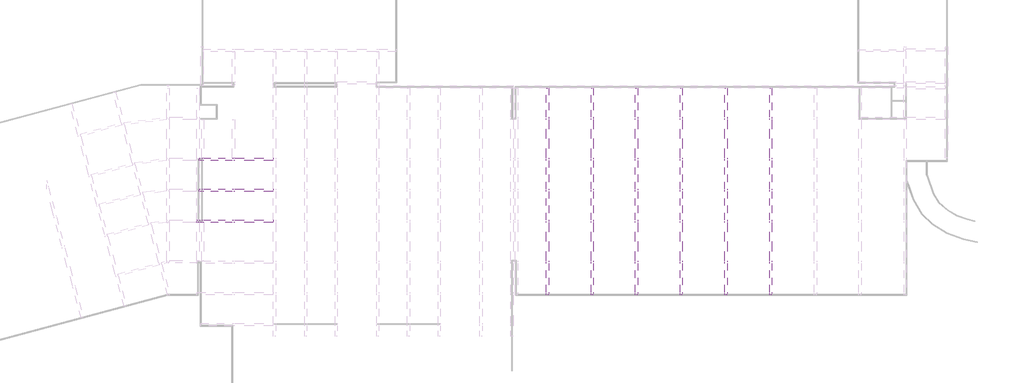
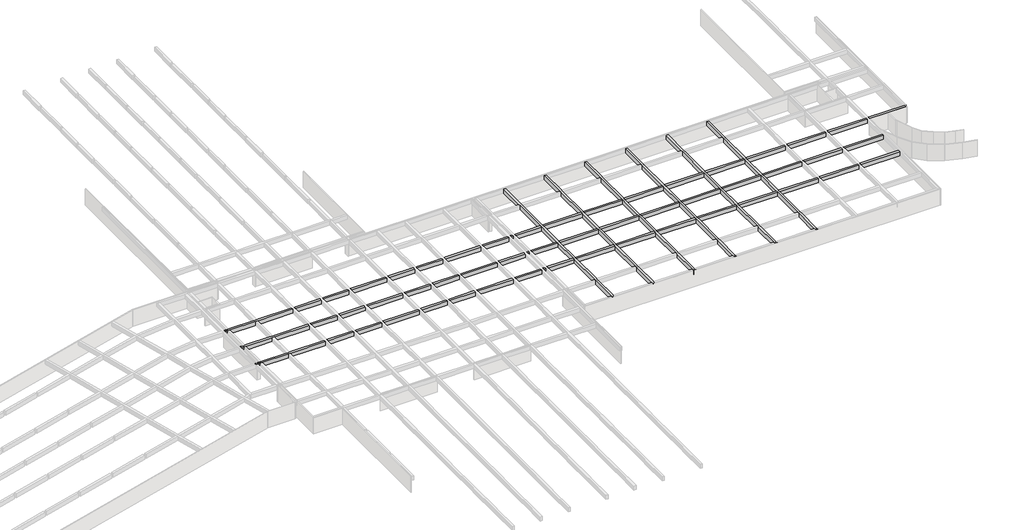
# One storey, part 9 of 14: 9 beams.
"""IFC4 building model written with IfcOpenShell, lengths in millimetres."""

from ifc_helpers import new_model, si_unit, origin, place, context, project, spatial, faceted_brep, element, save

model = new_model("IFC4")

# Units and contexts
model_context = context("Model", 3, world=origin())
ifc_project = project(units=[si_unit("LENGTHUNIT", "METRE", prefix="MILLI")], contexts=[model_context])

# Site, building, storey
site = spatial("IfcSite", under=ifc_project)
building = spatial("IfcBuilding", under=site)
storey = spatial("IfcBuildingStorey", under=building, Name="户型图", Elevation=0.0)

# Beams
placement = place(None, origin())
element("IfcBeam", 1, ObjectType="混凝土 - 矩形梁 : KL_beam", at=placement, inside=storey, context=model_context, shape_type="Brep", body=[
    faceted_brep([(73979.8514216, -218258.950757, 3300.0), (73579.8514216, -218258.950757, 3300.0), (73579.8514216, -218258.950757, 2500.0), (73979.8514216, -218258.950757, 2500.0), (73979.8514216, -218208.950757, 3300.0), (73979.8514216, -217808.950757, 3300.0), (73979.8514216, -212708.950757, 3300.0), (73979.8514216, -212308.950757, 3300.0), (73979.8514216, -205576.1028577, 3300.0), (73979.8514216, -205176.1028577, 3300.0), (73979.8514216, -200154.952508, 3300.0), (73979.8514216, -199754.952508, 3300.0), (73979.8514216, -194741.3993539, 3300.0), (73979.8514216, -194341.3993539, 3300.0), (73979.8514216, -187598.950757, 3300.0), (73979.8514216, -187198.950757, 3300.0), (73979.8514216, -182068.950757, 3300.0), (73579.8514216, -182068.950757, 3300.0), (73579.8514216, -187198.950757, 3300.0), (73579.8514216, -187598.950757, 3300.0), (73579.8514216, -194341.3993539, 3300.0), (73579.8514216, -194741.3993539, 3300.0), (73579.8514216, -199754.952508, 3300.0), (73579.8514216, -200154.952508, 3300.0), (73579.8514216, -205176.1028577, 3300.0), (73579.8514216, -205576.1028577, 3300.0), (73579.8514216, -212308.950757, 3300.0), (73579.8514216, -212708.950757, 3300.0), (73579.8514216, -217808.950757, 3300.0), (73579.8514216, -218208.950757, 3300.0), (73579.8514216, -182068.950757, 2500.0), (73579.8514216, -187198.950757, 2500.0), (73579.8514216, -187598.950757, 2500.0), (73579.8514216, -194341.3993539, 2500.0), (73579.8514216, -194741.3993539, 2500.0), (73579.8514216, -199754.952508, 2500.0), (73579.8514216, -200154.952508, 2500.0), (73579.8514216, -205176.1028577, 2500.0), (73579.8514216, -205576.1028577, 2500.0), (73579.8514216, -212308.950757, 2500.0), (73579.8514216, -212708.950757, 2500.0), (73579.8514216, -217808.950757, 2500.0), (73579.8514216, -218208.950757, 2500.0), (73979.8514216, -182068.950757, 2500.0), (73979.8514216, -187198.950757, 2500.0), (73979.8514216, -187598.950757, 2500.0), (73979.8514216, -194341.3993539, 2500.0), (73979.8514216, -194741.3993539, 2500.0), (73979.8514216, -199754.952508, 2500.0), (73979.8514216, -200154.952508, 2500.0), (73979.8514216, -205176.1028577, 2500.0), (73979.8514216, -205576.1028577, 2500.0), (73979.8514216, -212308.950757, 2500.0), (73979.8514216, -212708.950757, 2500.0), (73979.8514216, -217808.950757, 2500.0), (73979.8514216, -218208.950757, 2500.0)], [[[0, 1, 2, 3]], [[1, 0, 4, 5, 6, 7, 8, 9, 10, 11, 12, 13, 14, 15, 16, 17, 18, 19, 20, 21, 22, 23, 24, 25, 26, 27, 28, 29]], [[2, 1, 29, 28, 27, 26, 25, 24, 23, 22, 21, 20, 19, 18, 17, 30, 31, 32, 33, 34, 35, 36, 37, 38, 39, 40, 41, 42]], [[3, 2, 42, 41, 40, 39, 38, 37, 36, 35, 34, 33, 32, 31, 30, 43, 44, 45, 46, 47, 48, 49, 50, 51, 52, 53, 54, 55]], [[0, 3, 55, 54, 53, 52, 51, 50, 49, 48, 47, 46, 45, 44, 43, 16, 15, 14, 13, 12, 11, 10, 9, 8, 7, 6, 5, 4]], [[17, 16, 43, 30]]]),
])
element("IfcBeam", 2, ObjectType="混凝土 - 矩形梁 : KL_beam", at=placement, inside=storey, context=model_context, shape_type="Brep", body=[
    faceted_brep([(81379.8514216, -218258.950757, 3300.0), (81379.8514216, -218258.950757, 2500.0), (81779.8514216, -218258.950757, 2500.0), (81779.8514216, -218258.950757, 3300.0), (81779.8514216, -218208.950757, 3300.0), (81779.8514216, -217808.950757, 3300.0), (81779.8514216, -212708.950757, 3300.0), (81779.8514216, -212308.950757, 3300.0), (81779.8514216, -205576.1028577, 3300.0), (81779.8514216, -205176.1028577, 3300.0), (81779.8514216, -200154.952508, 3300.0), (81779.8514216, -199754.952508, 3300.0), (81779.8514216, -194741.3993539, 3300.0), (81779.8514216, -194341.3993539, 3300.0), (81779.8514216, -187598.950757, 3300.0), (81779.8514216, -187198.950757, 3300.0), (81779.8514216, -182068.950757, 3300.0), (81379.8514216, -182068.950757, 3300.0), (81379.8514216, -187198.950757, 3300.0), (81379.8514216, -187598.950757, 3300.0), (81379.8514216, -194341.3993539, 3300.0), (81379.8514216, -194741.3993539, 3300.0), (81379.8514216, -199754.952508, 3300.0), (81379.8514216, -200154.952508, 3300.0), (81379.8514216, -205176.1028577, 3300.0), (81379.8514216, -205576.1028577, 3300.0), (81379.8514216, -212308.950757, 3300.0), (81379.8514216, -212708.950757, 3300.0), (81379.8514216, -217808.950757, 3300.0), (81379.8514216, -218208.950757, 3300.0), (81779.8514216, -218208.950757, 2500.0), (81779.8514216, -217808.950757, 2500.0), (81779.8514216, -212708.950757, 2500.0), (81779.8514216, -212308.950757, 2500.0), (81779.8514216, -205576.1028577, 2500.0), (81779.8514216, -205176.1028577, 2500.0), (81779.8514216, -200154.952508, 2500.0), (81779.8514216, -199754.952508, 2500.0), (81779.8514216, -194741.3993539, 2500.0), (81779.8514216, -194341.3993539, 2500.0), (81779.8514216, -187598.950757, 2500.0), (81779.8514216, -187198.950757, 2500.0), (81779.8514216, -182068.950757, 2500.0), (81379.8514216, -218208.950757, 2500.0), (81379.8514216, -217808.950757, 2500.0), (81379.8514216, -212708.950757, 2500.0), (81379.8514216, -212308.950757, 2500.0), (81379.8514216, -205576.1028577, 2500.0), (81379.8514216, -205176.1028577, 2500.0), (81379.8514216, -200154.952508, 2500.0), (81379.8514216, -199754.952508, 2500.0), (81379.8514216, -194741.3993539, 2500.0), (81379.8514216, -194341.3993539, 2500.0), (81379.8514216, -187598.950757, 2500.0), (81379.8514216, -187198.950757, 2500.0), (81379.8514216, -182068.950757, 2500.0)], [[[0, 1, 2, 3]], [[0, 3, 4, 5, 6, 7, 8, 9, 10, 11, 12, 13, 14, 15, 16, 17, 18, 19, 20, 21, 22, 23, 24, 25, 26, 27, 28, 29]], [[3, 2, 30, 31, 32, 33, 34, 35, 36, 37, 38, 39, 40, 41, 42, 16, 15, 14, 13, 12, 11, 10, 9, 8, 7, 6, 5, 4]], [[2, 1, 43, 44, 45, 46, 47, 48, 49, 50, 51, 52, 53, 54, 55, 42, 41, 40, 39, 38, 37, 36, 35, 34, 33, 32, 31, 30]], [[1, 0, 29, 28, 27, 26, 25, 24, 23, 22, 21, 20, 19, 18, 17, 55, 54, 53, 52, 51, 50, 49, 48, 47, 46, 45, 44, 43]], [[17, 16, 42, 55]]]),
])
element("IfcBeam", 3, ObjectType="混凝土 - 矩形梁 : KL_beam", at=placement, inside=storey, context=model_context, shape_type="Brep", body=[
    faceted_brep([(89534.3329203, -218258.950757, 3300.0), (89134.3329203, -218258.950757, 3300.0), (89134.3329203, -218258.950757, 2500.0), (89534.3329203, -218258.950757, 2500.0), (89534.3329203, -218208.950757, 3300.0), (89534.3329203, -217808.950757, 3300.0), (89534.3329203, -212708.950757, 3300.0), (89534.3329203, -212308.950757, 3300.0), (89534.3329203, -205576.1028577, 3300.0), (89534.3329203, -205176.1028577, 3300.0), (89534.3329203, -200154.952508, 3300.0), (89534.3329203, -199754.952508, 3300.0), (89534.3329203, -194741.3993539, 3300.0), (89534.3329203, -194341.3993539, 3300.0), (89534.3329203, -187598.950757, 3300.0), (89534.3329203, -187198.950757, 3300.0), (89534.3329203, -182068.950757, 3300.0), (89134.3329203, -182068.950757, 3300.0), (89134.3329203, -187198.950757, 3300.0), (89134.3329203, -187598.950757, 3300.0), (89134.3329203, -194341.3993539, 3300.0), (89134.3329203, -194741.3993539, 3300.0), (89134.3329203, -199754.952508, 3300.0), (89134.3329203, -200154.952508, 3300.0), (89134.3329203, -205176.1028577, 3300.0), (89134.3329203, -205576.1028577, 3300.0), (89134.3329203, -212308.950757, 3300.0), (89134.3329203, -212708.950757, 3300.0), (89134.3329203, -217808.950757, 3300.0), (89134.3329203, -218208.950757, 3300.0), (89134.3329203, -182068.950757, 2500.0), (89134.3329203, -187198.950757, 2500.0), (89134.3329203, -187598.950757, 2500.0), (89134.3329203, -194341.3993539, 2500.0), (89134.3329203, -194741.3993539, 2500.0), (89134.3329203, -199754.952508, 2500.0), (89134.3329203, -200154.952508, 2500.0), (89134.3329203, -205176.1028577, 2500.0), (89134.3329203, -205576.1028577, 2500.0), (89134.3329203, -212308.950757, 2500.0), (89134.3329203, -212708.950757, 2500.0), (89134.3329203, -217808.950757, 2500.0), (89134.3329203, -218208.950757, 2500.0), (89534.3329203, -182068.950757, 2500.0), (89534.3329203, -187198.950757, 2500.0), (89534.3329203, -187598.950757, 2500.0), (89534.3329203, -194341.3993539, 2500.0), (89534.3329203, -194741.3993539, 2500.0), (89534.3329203, -199754.952508, 2500.0), (89534.3329203, -200154.952508, 2500.0), (89534.3329203, -205176.1028577, 2500.0), (89534.3329203, -205576.1028577, 2500.0), (89534.3329203, -212308.950757, 2500.0), (89534.3329203, -212708.950757, 2500.0), (89534.3329203, -217808.950757, 2500.0), (89534.3329203, -218208.950757, 2500.0)], [[[0, 1, 2, 3]], [[1, 0, 4, 5, 6, 7, 8, 9, 10, 11, 12, 13, 14, 15, 16, 17, 18, 19, 20, 21, 22, 23, 24, 25, 26, 27, 28, 29]], [[2, 1, 29, 28, 27, 26, 25, 24, 23, 22, 21, 20, 19, 18, 17, 30, 31, 32, 33, 34, 35, 36, 37, 38, 39, 40, 41, 42]], [[3, 2, 42, 41, 40, 39, 38, 37, 36, 35, 34, 33, 32, 31, 30, 43, 44, 45, 46, 47, 48, 49, 50, 51, 52, 53, 54, 55]], [[0, 3, 55, 54, 53, 52, 51, 50, 49, 48, 47, 46, 45, 44, 43, 16, 15, 14, 13, 12, 11, 10, 9, 8, 7, 6, 5, 4]], [[17, 16, 43, 30]]]),
])
element("IfcBeam", 4, ObjectType="混凝土 - 矩形梁 : KL_beam", at=placement, inside=storey, context=model_context, shape_type="Brep", body=[
    faceted_brep([(96934.3329203, -218258.950757, 3300.0), (96934.3329203, -218258.950757, 2500.0), (97334.3329203, -218258.950757, 2500.0), (97334.3329203, -218258.950757, 3300.0), (97334.3329203, -218208.950757, 3300.0), (97334.3329203, -217808.950757, 3300.0), (97334.3329203, -212708.950757, 3300.0), (97334.3329203, -212308.950757, 3300.0), (97334.3329203, -205576.1028577, 3300.0), (97334.3329203, -205176.1028577, 3300.0), (97334.3329203, -200154.952508, 3300.0), (97334.3329203, -199754.952508, 3300.0), (97334.3329203, -194741.3993539, 3300.0), (97334.3329203, -194341.3993539, 3300.0), (97334.3329203, -187598.950757, 3300.0), (97334.3329203, -187198.950757, 3300.0), (97334.3329203, -182068.950757, 3300.0), (96934.3329203, -182068.950757, 3300.0), (96934.3329203, -187198.950757, 3300.0), (96934.3329203, -187598.950757, 3300.0), (96934.3329203, -194341.3993539, 3300.0), (96934.3329203, -194741.3993539, 3300.0), (96934.3329203, -199754.952508, 3300.0), (96934.3329203, -200154.952508, 3300.0), (96934.3329203, -205176.1028577, 3300.0), (96934.3329203, -205576.1028577, 3300.0), (96934.3329203, -212308.950757, 3300.0), (96934.3329203, -212708.950757, 3300.0), (96934.3329203, -217808.950757, 3300.0), (96934.3329203, -218208.950757, 3300.0), (97334.3329203, -218208.950757, 2500.0), (97334.3329203, -217808.950757, 2500.0), (97334.3329203, -212708.950757, 2500.0), (97334.3329203, -212308.950757, 2500.0), (97334.3329203, -205576.1028577, 2500.0), (97334.3329203, -205176.1028577, 2500.0), (97334.3329203, -200154.952508, 2500.0), (97334.3329203, -199754.952508, 2500.0), (97334.3329203, -194741.3993539, 2500.0), (97334.3329203, -194341.3993539, 2500.0), (97334.3329203, -187598.950757, 2500.0), (97334.3329203, -187198.950757, 2500.0), (97334.3329203, -182068.950757, 2500.0), (96934.3329203, -218208.950757, 2500.0), (96934.3329203, -217808.950757, 2500.0), (96934.3329203, -212708.950757, 2500.0), (96934.3329203, -212308.950757, 2500.0), (96934.3329203, -205576.1028577, 2500.0), (96934.3329203, -205176.1028577, 2500.0), (96934.3329203, -200154.952508, 2500.0), (96934.3329203, -199754.952508, 2500.0), (96934.3329203, -194741.3993539, 2500.0), (96934.3329203, -194341.3993539, 2500.0), (96934.3329203, -187598.950757, 2500.0), (96934.3329203, -187198.950757, 2500.0), (96934.3329203, -182068.950757, 2500.0)], [[[0, 1, 2, 3]], [[0, 3, 4, 5, 6, 7, 8, 9, 10, 11, 12, 13, 14, 15, 16, 17, 18, 19, 20, 21, 22, 23, 24, 25, 26, 27, 28, 29]], [[3, 2, 30, 31, 32, 33, 34, 35, 36, 37, 38, 39, 40, 41, 42, 16, 15, 14, 13, 12, 11, 10, 9, 8, 7, 6, 5, 4]], [[2, 1, 43, 44, 45, 46, 47, 48, 49, 50, 51, 52, 53, 54, 55, 42, 41, 40, 39, 38, 37, 36, 35, 34, 33, 32, 31, 30]], [[1, 0, 29, 28, 27, 26, 25, 24, 23, 22, 21, 20, 19, 18, 17, 55, 54, 53, 52, 51, 50, 49, 48, 47, 46, 45, 44, 43]], [[17, 16, 42, 55]]]),
])
element("IfcBeam", 5, ObjectType="混凝土 - 矩形梁 : KL_beam", at=placement, inside=storey, context=model_context, shape_type="Brep", body=[
    faceted_brep([(105134.3329203, -218258.950757, 3300.0), (104734.3329203, -218258.950757, 3300.0), (104734.3329203, -218258.950757, 2500.0), (105134.3329203, -218258.950757, 2500.0), (105134.3329203, -218208.950757, 3300.0), (105134.3329203, -217808.950757, 3300.0), (105134.3329203, -212708.950757, 3300.0), (105134.3329203, -212308.950757, 3300.0), (105134.3329203, -205576.1028577, 3300.0), (105134.3329203, -205176.1028577, 3300.0), (105134.3329203, -200154.952508, 3300.0), (105134.3329203, -199754.952508, 3300.0), (105134.3329203, -194741.3993539, 3300.0), (105134.3329203, -194341.3993539, 3300.0), (105134.3329203, -187598.950757, 3300.0), (105134.3329203, -187198.950757, 3300.0), (105134.3329203, -182068.950757, 3300.0), (104734.3329203, -182068.950757, 3300.0), (104734.3329203, -187198.950757, 3300.0), (104734.3329203, -187598.950757, 3300.0), (104734.3329203, -194341.3993539, 3300.0), (104734.3329203, -194741.3993539, 3300.0), (104734.3329203, -199754.952508, 3300.0), (104734.3329203, -200154.952508, 3300.0), (104734.3329203, -205176.1028577, 3300.0), (104734.3329203, -205576.1028577, 3300.0), (104734.3329203, -212308.950757, 3300.0), (104734.3329203, -212708.950757, 3300.0), (104734.3329203, -217808.950757, 3300.0), (104734.3329203, -218208.950757, 3300.0), (104734.3329203, -182068.950757, 2500.0), (104734.3329203, -187198.950757, 2500.0), (104734.3329203, -187598.950757, 2500.0), (104734.3329203, -194341.3993539, 2500.0), (104734.3329203, -194741.3993539, 2500.0), (104734.3329203, -199754.952508, 2500.0), (104734.3329203, -200154.952508, 2500.0), (104734.3329203, -205176.1028577, 2500.0), (104734.3329203, -205576.1028577, 2500.0), (104734.3329203, -212308.950757, 2500.0), (104734.3329203, -212708.950757, 2500.0), (104734.3329203, -217808.950757, 2500.0), (104734.3329203, -218208.950757, 2500.0), (105134.3329203, -182068.950757, 2500.0), (105134.3329203, -187198.950757, 2500.0), (105134.3329203, -187598.950757, 2500.0), (105134.3329203, -194341.3993539, 2500.0), (105134.3329203, -194741.3993539, 2500.0), (105134.3329203, -199754.952508, 2500.0), (105134.3329203, -200154.952508, 2500.0), (105134.3329203, -205176.1028577, 2500.0), (105134.3329203, -205576.1028577, 2500.0), (105134.3329203, -212308.950757, 2500.0), (105134.3329203, -212708.950757, 2500.0), (105134.3329203, -217808.950757, 2500.0), (105134.3329203, -218208.950757, 2500.0)], [[[0, 1, 2, 3]], [[1, 0, 4, 5, 6, 7, 8, 9, 10, 11, 12, 13, 14, 15, 16, 17, 18, 19, 20, 21, 22, 23, 24, 25, 26, 27, 28, 29]], [[2, 1, 29, 28, 27, 26, 25, 24, 23, 22, 21, 20, 19, 18, 17, 30, 31, 32, 33, 34, 35, 36, 37, 38, 39, 40, 41, 42]], [[3, 2, 42, 41, 40, 39, 38, 37, 36, 35, 34, 33, 32, 31, 30, 43, 44, 45, 46, 47, 48, 49, 50, 51, 52, 53, 54, 55]], [[0, 3, 55, 54, 53, 52, 51, 50, 49, 48, 47, 46, 45, 44, 43, 16, 15, 14, 13, 12, 11, 10, 9, 8, 7, 6, 5, 4]], [[17, 16, 43, 30]]]),
])
element("IfcBeam", 6, ObjectType="混凝土 - 矩形梁 : KL_beam", at=placement, inside=storey, context=model_context, shape_type="Brep", body=[
    faceted_brep([(112555.6695954, -218258.950757, 3300.0), (112555.6695954, -218258.950757, 2500.0), (112955.6695954, -218258.950757, 2500.0), (112955.6695954, -218258.950757, 3300.0), (112955.6695954, -218208.950757, 3300.0), (112955.6695954, -217808.950757, 3300.0), (112955.6695954, -212708.950757, 3300.0), (112955.6695954, -212308.950757, 3300.0), (112955.6695954, -205576.1028577, 3300.0), (112955.6695954, -205176.1028577, 3300.0), (112955.6695954, -200154.952508, 3300.0), (112955.6695954, -199754.952508, 3300.0), (112955.6695954, -194741.3993539, 3300.0), (112955.6695954, -194341.3993539, 3300.0), (112955.6695954, -187598.950757, 3300.0), (112955.6695954, -187198.950757, 3300.0), (112955.6695954, -182068.950757, 3300.0), (112555.6695954, -182068.950757, 3300.0), (112555.6695954, -187198.950757, 3300.0), (112555.6695954, -187598.950757, 3300.0), (112555.6695954, -194341.3993539, 3300.0), (112555.6695954, -194741.3993539, 3300.0), (112555.6695954, -199754.952508, 3300.0), (112555.6695954, -200154.952508, 3300.0), (112555.6695954, -205176.1028577, 3300.0), (112555.6695954, -205576.1028577, 3300.0), (112555.6695954, -212308.950757, 3300.0), (112555.6695954, -212708.950757, 3300.0), (112555.6695954, -217808.950757, 3300.0), (112555.6695954, -218208.950757, 3300.0), (112955.6695954, -218208.950757, 2500.0), (112955.6695954, -217808.950757, 2500.0), (112955.6695954, -212708.950757, 2500.0), (112955.6695954, -212308.950757, 2500.0), (112955.6695954, -205576.1028577, 2500.0), (112955.6695954, -205176.1028577, 2500.0), (112955.6695954, -200154.952508, 2500.0), (112955.6695954, -199754.952508, 2500.0), (112955.6695954, -194741.3993539, 2500.0), (112955.6695954, -194341.3993539, 2500.0), (112955.6695954, -187598.950757, 2500.0), (112955.6695954, -187198.950757, 2500.0), (112955.6695954, -182068.950757, 2500.0), (112555.6695954, -218208.950757, 2500.0), (112555.6695954, -217808.950757, 2500.0), (112555.6695954, -212708.950757, 2500.0), (112555.6695954, -212308.950757, 2500.0), (112555.6695954, -205576.1028577, 2500.0), (112555.6695954, -205176.1028577, 2500.0), (112555.6695954, -200154.952508, 2500.0), (112555.6695954, -199754.952508, 2500.0), (112555.6695954, -194741.3993539, 2500.0), (112555.6695954, -194341.3993539, 2500.0), (112555.6695954, -187598.950757, 2500.0), (112555.6695954, -187198.950757, 2500.0), (112555.6695954, -182068.950757, 2500.0)], [[[0, 1, 2, 3]], [[0, 3, 4, 5, 6, 7, 8, 9, 10, 11, 12, 13, 14, 15, 16, 17, 18, 19, 20, 21, 22, 23, 24, 25, 26, 27, 28, 29]], [[3, 2, 30, 31, 32, 33, 34, 35, 36, 37, 38, 39, 40, 41, 42, 16, 15, 14, 13, 12, 11, 10, 9, 8, 7, 6, 5, 4]], [[2, 1, 43, 44, 45, 46, 47, 48, 49, 50, 51, 52, 53, 54, 55, 42, 41, 40, 39, 38, 37, 36, 35, 34, 33, 32, 31, 30]], [[1, 0, 29, 28, 27, 26, 25, 24, 23, 22, 21, 20, 19, 18, 17, 55, 54, 53, 52, 51, 50, 49, 48, 47, 46, 45, 44, 43]], [[17, 16, 42, 55]]]),
])
element("IfcBeam", 7, ObjectType="混凝土 - 矩形梁 : KL_beam", at=placement, inside=storey, context=model_context, shape_type="Brep", body=[
    faceted_brep([(25921.5607309, -194741.3993539, 3300.0), (25921.5607309, -194341.3993539, 3300.0), (19160.0865653, -194341.3993539, 3300.0), (18760.0865653, -194341.3993539, 3300.0), (13777.4621399, -194341.3993539, 3300.0), (13377.4621399, -194341.3993539, 3300.0), (12933.1378826, -194341.3993539, 3300.0), (12933.1378826, -194741.3993539, 3300.0), (13377.4621399, -194741.3993539, 3300.0), (13777.4621399, -194741.3993539, 3300.0), (18760.0865653, -194741.3993539, 3300.0), (19160.0865653, -194741.3993539, 3300.0), (25921.5607309, -194741.3993539, 2500.0), (12933.1378826, -194741.3993539, 2500.0), (13377.4621399, -194741.3993539, 2500.0), (13777.4621399, -194741.3993539, 2500.0), (18760.0865653, -194741.3993539, 2500.0), (19160.0865653, -194741.3993539, 2500.0), (25921.5607309, -194341.3993539, 2500.0), (12933.1378826, -194341.3993539, 2500.0), (13377.4621399, -194341.3993539, 2500.0), (13777.4621399, -194341.3993539, 2500.0), (18760.0865653, -194341.3993539, 2500.0), (19160.0865653, -194341.3993539, 2500.0)], [[[0, 1, 2, 3, 4, 5, 6, 7, 8, 9, 10, 11]], [[12, 0, 11, 10, 9, 8, 7, 13, 14, 15, 16, 17]], [[18, 12, 17, 16, 15, 14, 13, 19, 20, 21, 22, 23]], [[1, 18, 23, 22, 21, 20, 19, 6, 5, 4, 3, 2]], [[1, 0, 12, 18]], [[7, 6, 19, 13]]]),
    faceted_brep([(26321.5607309, -194741.3993539, 3300.0), (26321.5607309, -194341.3993539, 3300.0), (26321.5607309, -194341.3993539, 2500.0), (26321.5607309, -194741.3993539, 2500.0), (31351.9066405, -194341.3993539, 3300.0), (31351.9066405, -194741.3993539, 3300.0), (31351.9066405, -194741.3993539, 2500.0), (31351.9066405, -194341.3993539, 2500.0)], [[[0, 1, 2, 3]], [[4, 5, 6, 7]], [[1, 0, 5, 4]], [[0, 3, 6, 5]], [[3, 2, 7, 6]], [[2, 1, 4, 7]]]),
    faceted_brep([(31751.9066405, -194341.3993539, 3300.0), (31751.9066405, -194741.3993539, 3300.0), (36681.5607309, -194741.3993539, 3300.0), (36681.5607309, -194341.3993539, 3300.0), (31751.9066405, -194741.3993539, 2500.0), (36681.5607309, -194741.3993539, 2500.0), (31751.9066405, -194341.3993539, 2500.0), (36681.5607309, -194341.3993539, 2500.0)], [[[0, 1, 2, 3]], [[1, 4, 5, 2]], [[4, 6, 7, 5]], [[6, 0, 3, 7]], [[1, 0, 6, 4]], [[3, 2, 5, 7]]]),
    faceted_brep([(37081.5607309, -194741.3993539, 3300.0), (37081.5607309, -194341.3993539, 3300.0), (37081.5607309, -194341.3993539, 2500.0), (37081.5607309, -194741.3993539, 2500.0), (43931.9066405, -194341.3993539, 3300.0), (43931.9066405, -194741.3993539, 3300.0), (43931.9066405, -194741.3993539, 2500.0), (43931.9066405, -194341.3993539, 2500.0)], [[[0, 1, 2, 3]], [[4, 5, 6, 7]], [[1, 0, 5, 4]], [[0, 3, 6, 5]], [[3, 2, 7, 6]], [[2, 1, 4, 7]]]),
    faceted_brep([(44331.9066405, -194741.3993539, 3300.0), (44331.9066405, -194341.3993539, 3300.0), (44331.9066405, -194341.3993539, 2500.0), (44331.9066405, -194741.3993539, 2500.0), (49289.9831968, -194341.3993539, 3300.0), (49289.9831968, -194741.3993539, 3300.0), (49289.9831968, -194741.3993539, 2500.0), (49289.9831968, -194341.3993539, 2500.0)], [[[0, 1, 2, 3]], [[4, 5, 6, 7]], [[1, 0, 5, 4]], [[0, 3, 6, 5]], [[3, 2, 7, 6]], [[2, 1, 4, 7]]]),
    faceted_brep([(49689.9831968, -194741.3993539, 3300.0), (49689.9831968, -194341.3993539, 3300.0), (49689.9831968, -194341.3993539, 2500.0), (49689.9831968, -194741.3993539, 2500.0), (54689.9831968, -194341.3993539, 3300.0), (54689.9831968, -194741.3993539, 3300.0), (54689.9831968, -194741.3993539, 2500.0), (54689.9831968, -194341.3993539, 2500.0)], [[[0, 1, 2, 3]], [[4, 5, 6, 7]], [[1, 0, 5, 4]], [[0, 3, 6, 5]], [[3, 2, 7, 6]], [[2, 1, 4, 7]]]),
    faceted_brep([(55089.9831968, -194741.3993539, 3300.0), (55089.9831968, -194341.3993539, 3300.0), (55089.9831968, -194341.3993539, 2500.0), (55089.9831968, -194741.3993539, 2500.0), (61967.2949044, -194341.3993539, 3300.0), (61967.2949044, -194741.3993539, 3300.0), (61967.2949044, -194741.3993539, 2500.0), (61967.2949044, -194341.3993539, 2500.0)], [[[0, 1, 2, 3]], [[4, 5, 6, 7]], [[1, 0, 5, 4]], [[0, 3, 6, 5]], [[3, 2, 7, 6]], [[2, 1, 4, 7]]]),
    faceted_brep([(62367.2949044, -194741.3993539, 3300.0), (62367.2949044, -194341.3993539, 3300.0), (62367.2949044, -194341.3993539, 2500.0), (62367.2949044, -194741.3993539, 2500.0), (67367.2949044, -194341.3993539, 3300.0), (67367.2949044, -194741.3993539, 3300.0), (67367.2949044, -194741.3993539, 2500.0), (67367.2949044, -194341.3993539, 2500.0)], [[[0, 1, 2, 3]], [[4, 5, 6, 7]], [[1, 0, 5, 4]], [[0, 3, 6, 5]], [[3, 2, 7, 6]], [[2, 1, 4, 7]]]),
    faceted_brep([(67767.2949044, -194741.3993539, 3300.0), (67767.2949044, -194341.3993539, 3300.0), (67767.2949044, -194341.3993539, 2500.0), (67767.2949044, -194741.3993539, 2500.0), (68177.2949044, -194341.3993539, 3300.0), (68177.2949044, -194741.3993539, 3300.0), (68177.2949044, -194741.3993539, 2500.0), (68177.2949044, -194341.3993539, 2500.0)], [[[0, 1, 2, 3]], [[4, 5, 6, 7]], [[1, 0, 5, 4]], [[0, 3, 6, 5]], [[3, 2, 7, 6]], [[2, 1, 4, 7]]]),
    faceted_brep([(68577.2949044, -194741.3993539, 3300.0), (68577.2949044, -194341.3993539, 3300.0), (68577.2949044, -194341.3993539, 2500.0), (68577.2949044, -194741.3993539, 2500.0), (73579.8514216, -194341.3993539, 3300.0), (73579.8514216, -194741.3993539, 3300.0), (73579.8514216, -194741.3993539, 2500.0), (73579.8514216, -194341.3993539, 2500.0)], [[[0, 1, 2, 3]], [[4, 5, 6, 7]], [[1, 0, 5, 4]], [[0, 3, 6, 5]], [[3, 2, 7, 6]], [[2, 1, 4, 7]]]),
    faceted_brep([(73979.8514216, -194741.3993539, 3300.0), (73979.8514216, -194341.3993539, 3300.0), (73979.8514216, -194341.3993539, 2500.0), (73979.8514216, -194741.3993539, 2500.0), (81379.8514216, -194341.3993539, 3300.0), (81379.8514216, -194741.3993539, 3300.0), (81379.8514216, -194741.3993539, 2500.0), (81379.8514216, -194341.3993539, 2500.0)], [[[0, 1, 2, 3]], [[4, 5, 6, 7]], [[1, 0, 5, 4]], [[0, 3, 6, 5]], [[3, 2, 7, 6]], [[2, 1, 4, 7]]]),
    faceted_brep([(81779.8514216, -194741.3993539, 3300.0), (81779.8514216, -194341.3993539, 3300.0), (81779.8514216, -194341.3993539, 2500.0), (81779.8514216, -194741.3993539, 2500.0), (89134.3329203, -194341.3993539, 3300.0), (89134.3329203, -194741.3993539, 3300.0), (89134.3329203, -194741.3993539, 2500.0), (89134.3329203, -194341.3993539, 2500.0)], [[[0, 1, 2, 3]], [[4, 5, 6, 7]], [[1, 0, 5, 4]], [[0, 3, 6, 5]], [[3, 2, 7, 6]], [[2, 1, 4, 7]]]),
    faceted_brep([(89534.3329203, -194741.3993539, 3300.0), (89534.3329203, -194341.3993539, 3300.0), (89534.3329203, -194341.3993539, 2500.0), (89534.3329203, -194741.3993539, 2500.0), (96934.3329203, -194341.3993539, 3300.0), (96934.3329203, -194741.3993539, 3300.0), (96934.3329203, -194741.3993539, 2500.0), (96934.3329203, -194341.3993539, 2500.0)], [[[0, 1, 2, 3]], [[4, 5, 6, 7]], [[1, 0, 5, 4]], [[0, 3, 6, 5]], [[3, 2, 7, 6]], [[2, 1, 4, 7]]]),
    faceted_brep([(97334.3329203, -194741.3993539, 3300.0), (97334.3329203, -194341.3993539, 3300.0), (97334.3329203, -194341.3993539, 2500.0), (97334.3329203, -194741.3993539, 2500.0), (104734.3329203, -194341.3993539, 3300.0), (104734.3329203, -194741.3993539, 3300.0), (104734.3329203, -194741.3993539, 2500.0), (104734.3329203, -194341.3993539, 2500.0)], [[[0, 1, 2, 3]], [[4, 5, 6, 7]], [[1, 0, 5, 4]], [[0, 3, 6, 5]], [[3, 2, 7, 6]], [[2, 1, 4, 7]]]),
    faceted_brep([(105134.3329203, -194741.3993539, 3300.0), (105134.3329203, -194341.3993539, 3300.0), (105134.3329203, -194341.3993539, 2500.0), (105134.3329203, -194741.3993539, 2500.0), (112555.6695954, -194341.3993539, 3300.0), (112555.6695954, -194741.3993539, 3300.0), (112555.6695954, -194741.3993539, 2500.0), (112555.6695954, -194341.3993539, 2500.0)], [[[0, 1, 2, 3]], [[4, 5, 6, 7]], [[1, 0, 5, 4]], [[0, 3, 6, 5]], [[3, 2, 7, 6]], [[2, 1, 4, 7]]]),
    faceted_brep([(112955.6695954, -194741.3993539, 3300.0), (112955.6695954, -194341.3993539, 3300.0), (112955.6695954, -194341.3993539, 2500.0), (112955.6695954, -194741.3993539, 2500.0), (120367.2949044, -194341.3993539, 3300.0), (120367.2949044, -194741.3993539, 3300.0), (120367.2949044, -194741.3993539, 2500.0), (120367.2949044, -194341.3993539, 2500.0)], [[[0, 1, 2, 3]], [[4, 5, 6, 7]], [[1, 0, 5, 4]], [[0, 3, 6, 5]], [[3, 2, 7, 6]], [[2, 1, 4, 7]]]),
    faceted_brep([(120767.2949044, -194741.3993539, 3300.0), (120767.2949044, -194341.3993539, 3300.0), (120767.2949044, -194341.3993539, 2500.0), (120767.2949044, -194741.3993539, 2500.0), (128149.172254, -194341.3993539, 3300.0), (128149.172254, -194741.3993539, 3300.0), (128149.172254, -194741.3993539, 2500.0), (128149.172254, -194341.3993539, 2500.0)], [[[0, 1, 2, 3]], [[4, 5, 6, 7]], [[1, 0, 5, 4]], [[0, 3, 6, 5]], [[3, 2, 7, 6]], [[2, 1, 4, 7]]]),
    faceted_brep([(128549.172254, -194741.3993539, 3300.0), (128549.172254, -194341.3993539, 3300.0), (128549.172254, -194341.3993539, 2500.0), (128549.172254, -194741.3993539, 2500.0), (136047.2949044, -194341.3993539, 3300.0), (136047.2949044, -194741.3993539, 3300.0), (136047.2949044, -194741.3993539, 2500.0), (136047.2949044, -194341.3993539, 2500.0)], [[[0, 1, 2, 3]], [[4, 5, 6, 7]], [[1, 0, 5, 4]], [[0, 3, 6, 5]], [[3, 2, 7, 6]], [[2, 1, 4, 7]]]),
    faceted_brep([(136447.2949044, -194741.3993539, 3300.0), (136447.2949044, -194341.3993539, 3300.0), (136447.2949044, -194341.3993539, 2500.0), (136447.2949044, -194741.3993539, 2500.0), (143627.2949044, -194341.3993539, 3300.0), (143627.2949044, -194741.3993539, 3300.0), (143627.2949044, -194741.3993539, 2500.0), (143627.2949044, -194341.3993539, 2500.0), (143227.2949044, -194341.3993539, 3300.0), (143227.2949044, -194341.3993539, 2500.0)], [[[0, 1, 2, 3]], [[4, 5, 6, 7]], [[5, 4, 8, 1, 0]], [[6, 5, 0, 3]], [[7, 6, 3, 2, 9]], [[4, 7, 9, 2, 1, 8]]]),
])
element("IfcBeam", 8, ObjectType="混凝土 - 矩形梁 : KL_beam", at=placement, inside=storey, context=model_context, shape_type="Brep", body=[
    faceted_brep([(128549.172254, -199754.952508, 3300.0), (128549.172254, -200154.952508, 3300.0), (136047.2949044, -200154.952508, 3300.0), (136047.2949044, -199754.952508, 3300.0), (128549.172254, -199754.952508, 2500.0), (136047.2949044, -199754.952508, 2500.0), (128549.172254, -200154.952508, 2500.0), (136047.2949044, -200154.952508, 2500.0)], [[[0, 1, 2, 3]], [[4, 0, 3, 5]], [[6, 4, 5, 7]], [[1, 6, 7, 2]], [[1, 0, 4, 6]], [[3, 2, 7, 5]]]),
    faceted_brep([(25921.5607309, -199754.952508, 3300.0), (25921.5607309, -200154.952508, 3300.0), (25921.5607309, -200154.952508, 2500.0), (25921.5607309, -199754.952508, 2500.0), (19160.0865653, -199754.952508, 3300.0), (18760.0865653, -199754.952508, 3300.0), (13777.4621399, -199754.952508, 3300.0), (13377.4621399, -199754.952508, 3300.0), (12933.1378826, -199754.952508, 3300.0), (12933.1378826, -200154.952508, 3300.0), (13377.4621399, -200154.952508, 3300.0), (13777.4621399, -200154.952508, 3300.0), (18760.0865653, -200154.952508, 3300.0), (19160.0865653, -200154.952508, 3300.0), (19160.0865653, -199754.952508, 2500.0), (18760.0865653, -199754.952508, 2500.0), (13777.4621399, -199754.952508, 2500.0), (13377.4621399, -199754.952508, 2500.0), (12933.1378826, -199754.952508, 2500.0), (19160.0865653, -200154.952508, 2500.0), (18760.0865653, -200154.952508, 2500.0), (13777.4621399, -200154.952508, 2500.0), (13377.4621399, -200154.952508, 2500.0), (12933.1378826, -200154.952508, 2500.0)], [[[0, 1, 2, 3]], [[1, 0, 4, 5, 6, 7, 8, 9, 10, 11, 12, 13]], [[0, 3, 14, 15, 16, 17, 18, 8, 7, 6, 5, 4]], [[3, 2, 19, 20, 21, 22, 23, 18, 17, 16, 15, 14]], [[2, 1, 13, 12, 11, 10, 9, 23, 22, 21, 20, 19]], [[9, 8, 18, 23]]]),
    faceted_brep([(26321.5607309, -200154.952508, 3300.0), (26321.5607309, -199754.952508, 3300.0), (26321.5607309, -199754.952508, 2500.0), (26321.5607309, -200154.952508, 2500.0), (31351.9066405, -199754.952508, 3300.0), (31351.9066405, -200154.952508, 3300.0), (31351.9066405, -200154.952508, 2500.0), (31351.9066405, -199754.952508, 2500.0)], [[[0, 1, 2, 3]], [[4, 5, 6, 7]], [[1, 0, 5, 4]], [[2, 1, 4, 7]], [[3, 2, 7, 6]], [[0, 3, 6, 5]]]),
    faceted_brep([(31751.9066405, -200154.952508, 3300.0), (31751.9066405, -199754.952508, 3300.0), (31751.9066405, -199754.952508, 2500.0), (31751.9066405, -200154.952508, 2500.0), (36681.5607309, -199754.952508, 3300.0), (36681.5607309, -200154.952508, 3300.0), (36681.5607309, -200154.952508, 2500.0), (36681.5607309, -199754.952508, 2500.0)], [[[0, 1, 2, 3]], [[4, 5, 6, 7]], [[1, 0, 5, 4]], [[2, 1, 4, 7]], [[3, 2, 7, 6]], [[0, 3, 6, 5]]]),
    faceted_brep([(37081.5607309, -200154.952508, 3300.0), (37081.5607309, -199754.952508, 3300.0), (37081.5607309, -199754.952508, 2500.0), (37081.5607309, -200154.952508, 2500.0), (43931.9066405, -199754.952508, 3300.0), (43931.9066405, -200154.952508, 3300.0), (43931.9066405, -200154.952508, 2500.0), (43931.9066405, -199754.952508, 2500.0)], [[[0, 1, 2, 3]], [[4, 5, 6, 7]], [[1, 0, 5, 4]], [[2, 1, 4, 7]], [[3, 2, 7, 6]], [[0, 3, 6, 5]]]),
    faceted_brep([(44331.9066405, -200154.952508, 3300.0), (44331.9066405, -199754.952508, 3300.0), (44331.9066405, -199754.952508, 2500.0), (44331.9066405, -200154.952508, 2500.0), (49289.9831968, -199754.952508, 3300.0), (49289.9831968, -200154.952508, 3300.0), (49289.9831968, -200154.952508, 2500.0), (49289.9831968, -199754.952508, 2500.0)], [[[0, 1, 2, 3]], [[4, 5, 6, 7]], [[1, 0, 5, 4]], [[2, 1, 4, 7]], [[3, 2, 7, 6]], [[0, 3, 6, 5]]]),
    faceted_brep([(49689.9831968, -200154.952508, 3300.0), (49689.9831968, -199754.952508, 3300.0), (49689.9831968, -199754.952508, 2500.0), (49689.9831968, -200154.952508, 2500.0), (54689.9831968, -199754.952508, 3300.0), (54689.9831968, -200154.952508, 3300.0), (54689.9831968, -200154.952508, 2500.0), (54689.9831968, -199754.952508, 2500.0)], [[[0, 1, 2, 3]], [[4, 5, 6, 7]], [[1, 0, 5, 4]], [[2, 1, 4, 7]], [[3, 2, 7, 6]], [[0, 3, 6, 5]]]),
    faceted_brep([(55089.9831968, -200154.952508, 3300.0), (55089.9831968, -199754.952508, 3300.0), (55089.9831968, -199754.952508, 2500.0), (55089.9831968, -200154.952508, 2500.0), (61967.2949044, -199754.952508, 3300.0), (61967.2949044, -200154.952508, 3300.0), (61967.2949044, -200154.952508, 2500.0), (61967.2949044, -199754.952508, 2500.0)], [[[0, 1, 2, 3]], [[4, 5, 6, 7]], [[1, 0, 5, 4]], [[2, 1, 4, 7]], [[3, 2, 7, 6]], [[0, 3, 6, 5]]]),
    faceted_brep([(62367.2949044, -200154.952508, 3300.0), (62367.2949044, -199754.952508, 3300.0), (62367.2949044, -199754.952508, 2500.0), (62367.2949044, -200154.952508, 2500.0), (67367.2949044, -199754.952508, 3300.0), (67367.2949044, -200154.952508, 3300.0), (67367.2949044, -200154.952508, 2500.0), (67367.2949044, -199754.952508, 2500.0)], [[[0, 1, 2, 3]], [[4, 5, 6, 7]], [[1, 0, 5, 4]], [[2, 1, 4, 7]], [[3, 2, 7, 6]], [[0, 3, 6, 5]]]),
    faceted_brep([(67767.2949044, -200154.952508, 3300.0), (67767.2949044, -199754.952508, 3300.0), (67767.2949044, -199754.952508, 2500.0), (67767.2949044, -200154.952508, 2500.0), (68177.2949044, -199754.952508, 3300.0), (68177.2949044, -200154.952508, 3300.0), (68177.2949044, -200154.952508, 2500.0), (68177.2949044, -199754.952508, 2500.0)], [[[0, 1, 2, 3]], [[4, 5, 6, 7]], [[1, 0, 5, 4]], [[2, 1, 4, 7]], [[3, 2, 7, 6]], [[0, 3, 6, 5]]]),
    faceted_brep([(68577.2949044, -200154.952508, 3300.0), (68577.2949044, -199754.952508, 3300.0), (68577.2949044, -199754.952508, 2500.0), (68577.2949044, -200154.952508, 2500.0), (73579.8514216, -199754.952508, 3300.0), (73579.8514216, -200154.952508, 3300.0), (73579.8514216, -200154.952508, 2500.0), (73579.8514216, -199754.952508, 2500.0)], [[[0, 1, 2, 3]], [[4, 5, 6, 7]], [[1, 0, 5, 4]], [[2, 1, 4, 7]], [[3, 2, 7, 6]], [[0, 3, 6, 5]]]),
    faceted_brep([(73979.8514216, -200154.952508, 3300.0), (73979.8514216, -199754.952508, 3300.0), (73979.8514216, -199754.952508, 2500.0), (73979.8514216, -200154.952508, 2500.0), (81379.8514216, -199754.952508, 3300.0), (81379.8514216, -200154.952508, 3300.0), (81379.8514216, -200154.952508, 2500.0), (81379.8514216, -199754.952508, 2500.0)], [[[0, 1, 2, 3]], [[4, 5, 6, 7]], [[1, 0, 5, 4]], [[2, 1, 4, 7]], [[3, 2, 7, 6]], [[0, 3, 6, 5]]]),
    faceted_brep([(81779.8514216, -200154.952508, 3300.0), (81779.8514216, -199754.952508, 3300.0), (81779.8514216, -199754.952508, 2500.0), (81779.8514216, -200154.952508, 2500.0), (89134.3329203, -199754.952508, 3300.0), (89134.3329203, -200154.952508, 3300.0), (89134.3329203, -200154.952508, 2500.0), (89134.3329203, -199754.952508, 2500.0)], [[[0, 1, 2, 3]], [[4, 5, 6, 7]], [[1, 0, 5, 4]], [[2, 1, 4, 7]], [[3, 2, 7, 6]], [[0, 3, 6, 5]]]),
    faceted_brep([(89534.3329203, -200154.952508, 3300.0), (89534.3329203, -199754.952508, 3300.0), (89534.3329203, -199754.952508, 2500.0), (89534.3329203, -200154.952508, 2500.0), (96934.3329203, -199754.952508, 3300.0), (96934.3329203, -200154.952508, 3300.0), (96934.3329203, -200154.952508, 2500.0), (96934.3329203, -199754.952508, 2500.0)], [[[0, 1, 2, 3]], [[4, 5, 6, 7]], [[1, 0, 5, 4]], [[2, 1, 4, 7]], [[3, 2, 7, 6]], [[0, 3, 6, 5]]]),
    faceted_brep([(97334.3329203, -200154.952508, 3300.0), (97334.3329203, -199754.952508, 3300.0), (97334.3329203, -199754.952508, 2500.0), (97334.3329203, -200154.952508, 2500.0), (104734.3329203, -199754.952508, 3300.0), (104734.3329203, -200154.952508, 3300.0), (104734.3329203, -200154.952508, 2500.0), (104734.3329203, -199754.952508, 2500.0)], [[[0, 1, 2, 3]], [[4, 5, 6, 7]], [[1, 0, 5, 4]], [[2, 1, 4, 7]], [[3, 2, 7, 6]], [[0, 3, 6, 5]]]),
    faceted_brep([(105134.3329203, -200154.952508, 3300.0), (105134.3329203, -199754.952508, 3300.0), (105134.3329203, -199754.952508, 2500.0), (105134.3329203, -200154.952508, 2500.0), (112555.6695954, -199754.952508, 3300.0), (112555.6695954, -200154.952508, 3300.0), (112555.6695954, -200154.952508, 2500.0), (112555.6695954, -199754.952508, 2500.0)], [[[0, 1, 2, 3]], [[4, 5, 6, 7]], [[1, 0, 5, 4]], [[2, 1, 4, 7]], [[3, 2, 7, 6]], [[0, 3, 6, 5]]]),
    faceted_brep([(112955.6695954, -200154.952508, 3300.0), (112955.6695954, -199754.952508, 3300.0), (112955.6695954, -199754.952508, 2500.0), (112955.6695954, -200154.952508, 2500.0), (120367.2949044, -199754.952508, 3300.0), (120367.2949044, -200154.952508, 3300.0), (120367.2949044, -200154.952508, 2500.0), (120367.2949044, -199754.952508, 2500.0)], [[[0, 1, 2, 3]], [[4, 5, 6, 7]], [[1, 0, 5, 4]], [[2, 1, 4, 7]], [[3, 2, 7, 6]], [[0, 3, 6, 5]]]),
    faceted_brep([(120767.2949044, -200154.952508, 3300.0), (120767.2949044, -199754.952508, 3300.0), (120767.2949044, -199754.952508, 2500.0), (120767.2949044, -200154.952508, 2500.0), (128149.172254, -199754.952508, 3300.0), (128149.172254, -200154.952508, 3300.0), (128149.172254, -200154.952508, 2500.0), (128149.172254, -199754.952508, 2500.0)], [[[0, 1, 2, 3]], [[4, 5, 6, 7]], [[1, 0, 5, 4]], [[2, 1, 4, 7]], [[3, 2, 7, 6]], [[0, 3, 6, 5]]]),
])
element("IfcBeam", 9, ObjectType="混凝土 - 矩形梁 : KL_beam", at=placement, inside=storey, context=model_context, shape_type="Brep", body=[
    faceted_brep([(25921.5607309, -205576.1028577, 3300.0), (25921.5607309, -205176.1028577, 3300.0), (19160.0865653, -205176.1028577, 3300.0), (18760.0865653, -205176.1028577, 3300.0), (13777.4621399, -205176.1028577, 3300.0), (13377.4621399, -205176.1028577, 3300.0), (12933.1378826, -205176.1028577, 3300.0), (12533.1378826, -205176.1028577, 3300.0), (12533.1378826, -205576.1028577, 3300.0), (12933.1378826, -205576.1028577, 3300.0), (13377.4621399, -205576.1028577, 3300.0), (13777.4621399, -205576.1028577, 3300.0), (18760.0865653, -205576.1028577, 3300.0), (19160.0865653, -205576.1028577, 3300.0), (25921.5607309, -205576.1028577, 2500.0), (12533.1378826, -205576.1028577, 2500.0), (12933.1378826, -205576.1028577, 2500.0), (13377.4621399, -205576.1028577, 2500.0), (13777.4621399, -205576.1028577, 2500.0), (18760.0865653, -205576.1028577, 2500.0), (19160.0865653, -205576.1028577, 2500.0), (25921.5607309, -205176.1028577, 2500.0), (12533.1378826, -205176.1028577, 2500.0), (12933.1378826, -205176.1028577, 2500.0), (13377.4621399, -205176.1028577, 2500.0), (13777.4621399, -205176.1028577, 2500.0), (18760.0865653, -205176.1028577, 2500.0), (19160.0865653, -205176.1028577, 2500.0)], [[[0, 1, 2, 3, 4, 5, 6, 7, 8, 9, 10, 11, 12, 13]], [[14, 0, 13, 12, 11, 10, 9, 8, 15, 16, 17, 18, 19, 20]], [[21, 14, 20, 19, 18, 17, 16, 15, 22, 23, 24, 25, 26, 27]], [[1, 21, 27, 26, 25, 24, 23, 22, 7, 6, 5, 4, 3, 2]], [[1, 0, 14, 21]], [[8, 7, 22, 15]]]),
    faceted_brep([(26321.5607309, -205576.1028577, 3300.0), (26321.5607309, -205176.1028577, 3300.0), (26321.5607309, -205176.1028577, 2500.0), (26321.5607309, -205576.1028577, 2500.0), (31351.9066405, -205176.1028577, 3300.0), (31351.9066405, -205576.1028577, 3300.0), (31351.9066405, -205576.1028577, 2500.0), (31351.9066405, -205176.1028577, 2500.0)], [[[0, 1, 2, 3]], [[4, 5, 6, 7]], [[1, 0, 5, 4]], [[0, 3, 6, 5]], [[3, 2, 7, 6]], [[2, 1, 4, 7]]]),
    faceted_brep([(31751.9066405, -205176.1028577, 3300.0), (31751.9066405, -205576.1028577, 3300.0), (36681.5607309, -205576.1028577, 3300.0), (36681.5607309, -205176.1028577, 3300.0), (31751.9066405, -205576.1028577, 2500.0), (36681.5607309, -205576.1028577, 2500.0), (31751.9066405, -205176.1028577, 2500.0), (36681.5607309, -205176.1028577, 2500.0)], [[[0, 1, 2, 3]], [[1, 4, 5, 2]], [[4, 6, 7, 5]], [[6, 0, 3, 7]], [[1, 0, 6, 4]], [[3, 2, 5, 7]]]),
    faceted_brep([(37081.5607309, -205576.1028577, 3300.0), (37081.5607309, -205176.1028577, 3300.0), (37081.5607309, -205176.1028577, 2500.0), (37081.5607309, -205576.1028577, 2500.0), (43931.9066405, -205176.1028577, 3300.0), (43931.9066405, -205576.1028577, 3300.0), (43931.9066405, -205576.1028577, 2500.0), (43931.9066405, -205176.1028577, 2500.0)], [[[0, 1, 2, 3]], [[4, 5, 6, 7]], [[1, 0, 5, 4]], [[0, 3, 6, 5]], [[3, 2, 7, 6]], [[2, 1, 4, 7]]]),
    faceted_brep([(44331.9066405, -205576.1028577, 3300.0), (44331.9066405, -205176.1028577, 3300.0), (44331.9066405, -205176.1028577, 2500.0), (44331.9066405, -205576.1028577, 2500.0), (49289.9831968, -205176.1028577, 3300.0), (49289.9831968, -205576.1028577, 3300.0), (49289.9831968, -205576.1028577, 2500.0), (49289.9831968, -205176.1028577, 2500.0)], [[[0, 1, 2, 3]], [[4, 5, 6, 7]], [[1, 0, 5, 4]], [[0, 3, 6, 5]], [[3, 2, 7, 6]], [[2, 1, 4, 7]]]),
    faceted_brep([(49689.9831968, -205576.1028577, 3300.0), (49689.9831968, -205176.1028577, 3300.0), (49689.9831968, -205176.1028577, 2500.0), (49689.9831968, -205576.1028577, 2500.0), (54689.9831968, -205176.1028577, 3300.0), (54689.9831968, -205576.1028577, 3300.0), (54689.9831968, -205576.1028577, 2500.0), (54689.9831968, -205176.1028577, 2500.0)], [[[0, 1, 2, 3]], [[4, 5, 6, 7]], [[1, 0, 5, 4]], [[0, 3, 6, 5]], [[3, 2, 7, 6]], [[2, 1, 4, 7]]]),
    faceted_brep([(55089.9831968, -205576.1028577, 3300.0), (55089.9831968, -205176.1028577, 3300.0), (55089.9831968, -205176.1028577, 2500.0), (55089.9831968, -205576.1028577, 2500.0), (61967.2949044, -205176.1028577, 3300.0), (61967.2949044, -205576.1028577, 3300.0), (61967.2949044, -205576.1028577, 2500.0), (61967.2949044, -205176.1028577, 2500.0)], [[[0, 1, 2, 3]], [[4, 5, 6, 7]], [[1, 0, 5, 4]], [[0, 3, 6, 5]], [[3, 2, 7, 6]], [[2, 1, 4, 7]]]),
    faceted_brep([(62367.2949044, -205576.1028577, 3300.0), (62367.2949044, -205176.1028577, 3300.0), (62367.2949044, -205176.1028577, 2500.0), (62367.2949044, -205576.1028577, 2500.0), (67367.2949044, -205176.1028577, 3300.0), (67367.2949044, -205576.1028577, 3300.0), (67367.2949044, -205576.1028577, 2500.0), (67367.2949044, -205176.1028577, 2500.0)], [[[0, 1, 2, 3]], [[4, 5, 6, 7]], [[1, 0, 5, 4]], [[0, 3, 6, 5]], [[3, 2, 7, 6]], [[2, 1, 4, 7]]]),
    faceted_brep([(67767.2949044, -205576.1028577, 3300.0), (67767.2949044, -205176.1028577, 3300.0), (67767.2949044, -205176.1028577, 2500.0), (67767.2949044, -205576.1028577, 2500.0), (68177.2949044, -205176.1028577, 3300.0), (68177.2949044, -205576.1028577, 3300.0), (68177.2949044, -205576.1028577, 2500.0), (68177.2949044, -205176.1028577, 2500.0)], [[[0, 1, 2, 3]], [[4, 5, 6, 7]], [[1, 0, 5, 4]], [[0, 3, 6, 5]], [[3, 2, 7, 6]], [[2, 1, 4, 7]]]),
    faceted_brep([(68577.2949044, -205576.1028577, 3300.0), (68577.2949044, -205176.1028577, 3300.0), (68577.2949044, -205176.1028577, 2500.0), (68577.2949044, -205576.1028577, 2500.0), (73579.8514216, -205176.1028577, 3300.0), (73579.8514216, -205576.1028577, 3300.0), (73579.8514216, -205576.1028577, 2500.0), (73579.8514216, -205176.1028577, 2500.0)], [[[0, 1, 2, 3]], [[4, 5, 6, 7]], [[1, 0, 5, 4]], [[0, 3, 6, 5]], [[3, 2, 7, 6]], [[2, 1, 4, 7]]]),
    faceted_brep([(73979.8514216, -205576.1028577, 3300.0), (73979.8514216, -205176.1028577, 3300.0), (73979.8514216, -205176.1028577, 2500.0), (73979.8514216, -205576.1028577, 2500.0), (81379.8514216, -205176.1028577, 3300.0), (81379.8514216, -205576.1028577, 3300.0), (81379.8514216, -205576.1028577, 2500.0), (81379.8514216, -205176.1028577, 2500.0)], [[[0, 1, 2, 3]], [[4, 5, 6, 7]], [[1, 0, 5, 4]], [[0, 3, 6, 5]], [[3, 2, 7, 6]], [[2, 1, 4, 7]]]),
    faceted_brep([(81779.8514216, -205576.1028577, 3300.0), (81779.8514216, -205176.1028577, 3300.0), (81779.8514216, -205176.1028577, 2500.0), (81779.8514216, -205576.1028577, 2500.0), (89134.3329203, -205176.1028577, 3300.0), (89134.3329203, -205576.1028577, 3300.0), (89134.3329203, -205576.1028577, 2500.0), (89134.3329203, -205176.1028577, 2500.0)], [[[0, 1, 2, 3]], [[4, 5, 6, 7]], [[1, 0, 5, 4]], [[0, 3, 6, 5]], [[3, 2, 7, 6]], [[2, 1, 4, 7]]]),
    faceted_brep([(89534.3329203, -205576.1028577, 3300.0), (89534.3329203, -205176.1028577, 3300.0), (89534.3329203, -205176.1028577, 2500.0), (89534.3329203, -205576.1028577, 2500.0), (96934.3329203, -205176.1028577, 3300.0), (96934.3329203, -205576.1028577, 3300.0), (96934.3329203, -205576.1028577, 2500.0), (96934.3329203, -205176.1028577, 2500.0)], [[[0, 1, 2, 3]], [[4, 5, 6, 7]], [[1, 0, 5, 4]], [[0, 3, 6, 5]], [[3, 2, 7, 6]], [[2, 1, 4, 7]]]),
    faceted_brep([(97334.3329203, -205576.1028577, 3300.0), (97334.3329203, -205176.1028577, 3300.0), (97334.3329203, -205176.1028577, 2500.0), (97334.3329203, -205576.1028577, 2500.0), (104734.3329203, -205176.1028577, 3300.0), (104734.3329203, -205576.1028577, 3300.0), (104734.3329203, -205576.1028577, 2500.0), (104734.3329203, -205176.1028577, 2500.0)], [[[0, 1, 2, 3]], [[4, 5, 6, 7]], [[1, 0, 5, 4]], [[0, 3, 6, 5]], [[3, 2, 7, 6]], [[2, 1, 4, 7]]]),
    faceted_brep([(105134.3329203, -205576.1028577, 3300.0), (105134.3329203, -205176.1028577, 3300.0), (105134.3329203, -205176.1028577, 2500.0), (105134.3329203, -205576.1028577, 2500.0), (112555.6695954, -205176.1028577, 3300.0), (112555.6695954, -205576.1028577, 3300.0), (112555.6695954, -205576.1028577, 2500.0), (112555.6695954, -205176.1028577, 2500.0)], [[[0, 1, 2, 3]], [[4, 5, 6, 7]], [[1, 0, 5, 4]], [[0, 3, 6, 5]], [[3, 2, 7, 6]], [[2, 1, 4, 7]]]),
    faceted_brep([(112955.6695954, -205576.1028577, 3300.0), (112955.6695954, -205176.1028577, 3300.0), (112955.6695954, -205176.1028577, 2500.0), (112955.6695954, -205576.1028577, 2500.0), (120367.2949044, -205176.1028577, 3300.0), (120367.2949044, -205576.1028577, 3300.0), (120367.2949044, -205576.1028577, 2500.0), (120367.2949044, -205176.1028577, 2500.0)], [[[0, 1, 2, 3]], [[4, 5, 6, 7]], [[1, 0, 5, 4]], [[0, 3, 6, 5]], [[3, 2, 7, 6]], [[2, 1, 4, 7]]]),
    faceted_brep([(120767.2949044, -205576.1028577, 3300.0), (120767.2949044, -205176.1028577, 3300.0), (120767.2949044, -205176.1028577, 2500.0), (120767.2949044, -205576.1028577, 2500.0), (128149.172254, -205176.1028577, 3300.0), (128149.172254, -205576.1028577, 3300.0), (128149.172254, -205576.1028577, 2500.0), (128149.172254, -205176.1028577, 2500.0)], [[[0, 1, 2, 3]], [[4, 5, 6, 7]], [[1, 0, 5, 4]], [[0, 3, 6, 5]], [[3, 2, 7, 6]], [[2, 1, 4, 7]]]),
    faceted_brep([(128549.172254, -205576.1028577, 3300.0), (128549.172254, -205176.1028577, 3300.0), (128549.172254, -205176.1028577, 2500.0), (128549.172254, -205576.1028577, 2500.0), (136047.2949044, -205176.1028577, 3300.0), (136047.2949044, -205576.1028577, 3300.0), (136047.2949044, -205576.1028577, 2500.0), (136047.2949044, -205176.1028577, 2500.0)], [[[0, 1, 2, 3]], [[4, 5, 6, 7]], [[1, 0, 5, 4]], [[0, 3, 6, 5]], [[3, 2, 7, 6]], [[2, 1, 4, 7]]]),
])

save(model, "model.ifc")

# Revit data of these elements
# Type "混凝土 - 矩形梁 : KL_beam"
#   Length [instance default] = 1524 mm
#   b = 400 mm
#   h = 800 mm
#   Structural Material [instance default] = 混凝土 - 现场浇注混凝土
#   Assembly Code = ""
# Elements 1, 2, 3, 4, 5, 6, 7, 8, 9 (IfcBeam, "混凝土 - 矩形梁 : KL_beam")
#   Comments = ""
#   Structural Material = none
#   Phase Created = 新构造
# Materials
#   "混凝土 - 现场浇注混凝土": class "混凝土", colour RGB 192 192 192, transparency 0
